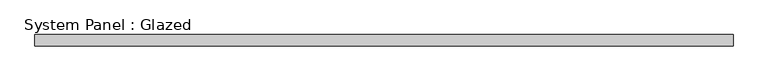
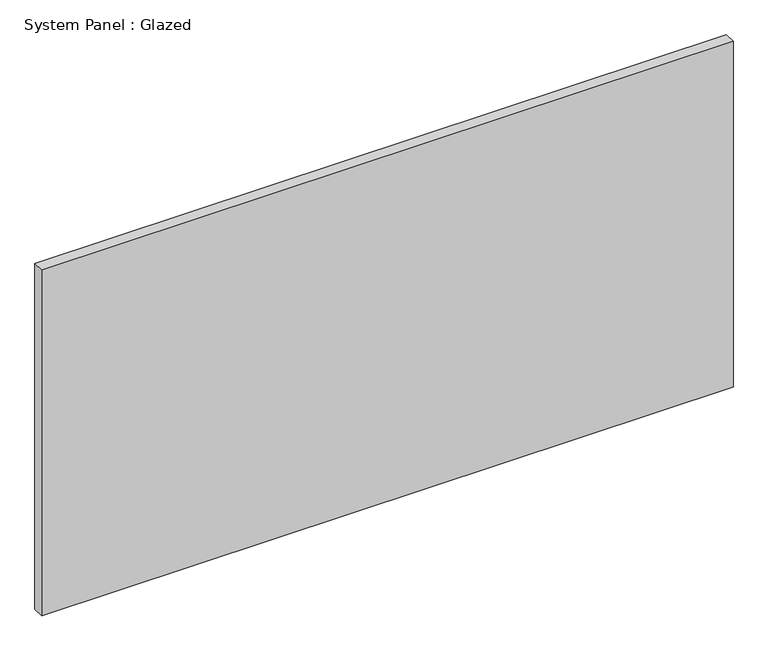
"""IFC4 building model written with IfcOpenShell, lengths in millimetres: plate geometry, System Panel : Glazed."""

import ifcopenshell
import ifcopenshell.guid

model = None  # the IFC model being written
_history = None  # IfcOwnerHistory: only IFC2X3 demands one
_inside = {}  # id of a spatial element -> (the spatial element, [elements in it])
_under = {}  # id of a project, library or spatial element -> (it, [spatial elements below it])
_declared = {}  # id of a project -> (the project, [libraries it declares])
_typed = {}  # id of a type object -> (the type object, [elements of that type])
_made_of = {}  # id of a material, layer set ... -> (it, [elements and type objects made of it])


def new_model(schema):
    """Start an empty IFC model of exactly this schema.

    Asked for "IFC4X3", IfcOpenShell would pick the latest addendum, in which some entities
    have other attributes; the version numbers below select the first issue.
    IFC2X3 requires an IfcOwnerHistory on every rooted entity: one is made here for all.
    """
    global model, _history
    if schema == "IFC4X3":
        model = ifcopenshell.file(schema_version=(4, 3, 0, 0))
    else:
        model = ifcopenshell.file(schema=schema)
    _inside.clear()
    _under.clear()
    _declared.clear()
    _typed.clear()
    _made_of.clear()
    _history = None
    if model.schema == "IFC2X3":
        org = make("IfcOrganization", Name="unknown")
        user = make(
            "IfcPersonAndOrganization",
            ThePerson=make("IfcPerson", FamilyName="unknown"),
            TheOrganization=org,
        )
        app = make(
            "IfcApplication",
            ApplicationDeveloper=org,
            Version="unknown",
            ApplicationFullName="unknown",
            ApplicationIdentifier="unknown",
        )
        _history = make(
            "IfcOwnerHistory",
            OwningUser=user,
            OwningApplication=app,
            ChangeAction="ADDED",
            CreationDate=0,
        )
    return model


def make(cls, **values):
    """One entity of the class cls with the attributes given. An attribute that is None is left unset."""
    return model.create_entity(
        cls, **{name: value for name, value in values.items() if value is not None}
    )


def rooted(cls, **values):
    """An entity with a GlobalId (a new one), such as an element, a storey or a relation."""
    return make(cls, GlobalId=ifcopenshell.guid.new(), OwnerHistory=_history, **values)


def si_unit(unit_type, name, prefix=None):
    """IfcSIUnit, for example si_unit("LENGTHUNIT", "METRE", prefix="MILLI")."""
    return make("IfcSIUnit", UnitType=unit_type, Prefix=prefix, Name=name)


def assignment(units):
    """IfcUnitAssignment: the units of a project."""
    return None if units is None else make("IfcUnitAssignment", Units=units)


def point(xyz):
    """IfcCartesianPoint."""
    return None if xyz is None else make("IfcCartesianPoint", Coordinates=xyz)


def direction(xyz):
    """IfcDirection."""
    return None if xyz is None else make("IfcDirection", DirectionRatios=xyz)


def frame(location, z_axis=None, x_axis=None):
    """IfcAxis2Placement3D, a coordinate frame: its origin and axes. An axis left out is left unset."""
    return make(
        "IfcAxis2Placement3D",
        Location=point(location),
        Axis=direction(z_axis),
        RefDirection=direction(x_axis),
    )


def origin():
    """The frame at (0, 0, 0) with its axes left unset."""
    return frame((0.0, 0.0, 0.0))


def origin_with_axes():
    """The frame at (0, 0, 0) with the z axis (0, 0, 1) and the x axis (1, 0, 0) written out."""
    return frame((0.0, 0.0, 0.0), z_axis=(0.0, 0.0, 1.0), x_axis=(1.0, 0.0, 0.0))


def place(relative_to, where):
    """IfcLocalPlacement: puts the frame where relative to a parent placement (None: the world)."""
    return make(
        "IfcLocalPlacement", PlacementRelTo=relative_to, RelativePlacement=where
    )


def context(
    kind, dimensions, precision=None, world=None, true_north=None, identifier=None
):
    """IfcGeometricRepresentationContext, for example the 3D "Model" context."""
    return make(
        "IfcGeometricRepresentationContext",
        ContextIdentifier=identifier,
        ContextType=kind,
        CoordinateSpaceDimension=dimensions,
        Precision=precision,
        WorldCoordinateSystem=world,
        TrueNorth=true_north,
    )


def project(units=None, contexts=None):
    """IfcProject with its units and contexts."""
    return rooted(
        "IfcProject",
        Name="project",
        RepresentationContexts=contexts,
        UnitsInContext=assignment(units),
    )


def spatial(cls, under=None, at=None, **own):
    """A site, building, storey or space (cls), placed at a placement, below another one or the project."""
    s = rooted(cls, ObjectPlacement=at, **own)
    if under is not None:
        _under.setdefault(under.id(), (under, []))[1].append(s)
    return s


def polyline(points):
    """IfcPolyline through the points."""
    return make("IfcPolyline", Points=[point(p) for p in points])


def outline(outer, holes=None, kind="AREA"):
    """IfcArbitraryClosedProfileDef: a profile drawn as a closed curve; with holes, ...WithVoids."""
    if holes is None:
        return make("IfcArbitraryClosedProfileDef", ProfileType=kind, OuterCurve=outer)
    return make(
        "IfcArbitraryProfileDefWithVoids",
        ProfileType=kind,
        OuterCurve=outer,
        InnerCurves=holes,
    )


def extrude(swept, where, along, depth):
    """IfcExtrudedAreaSolid: the profile swept, set in the frame where, extruded along a direction by depth."""
    return make(
        "IfcExtrudedAreaSolid",
        SweptArea=swept,
        Position=where,
        ExtrudedDirection=direction(along),
        Depth=depth,
    )


def shape(context_of_items, identifier, shape_type, items):
    """IfcShapeRepresentation: the items that make up one representation, for example the "Body"."""
    return make(
        "IfcShapeRepresentation",
        ContextOfItems=context_of_items,
        RepresentationIdentifier=identifier,
        RepresentationType=shape_type,
        Items=items,
    )


def source(mapping_origin, context_of_items, identifier, shape_type, items):
    """IfcRepresentationMap: a shape defined once, which mapped items show again and again."""
    return make(
        "IfcRepresentationMap",
        MappingOrigin=mapping_origin,
        MappedRepresentation=shape(context_of_items, identifier, shape_type, items),
    )


def transform(
    local_origin,
    x_axis=None,
    y_axis=None,
    z_axis=None,
    scale=None,
    scale2=None,
    scale3=None,
    uniform=True,
):
    """IfcCartesianTransformationOperator3D, or its non-uniform kind. x_axis, y_axis, z_axis: its Axis1, 2, 3."""
    if uniform:
        return make(
            "IfcCartesianTransformationOperator3D",
            Axis1=direction(x_axis),
            Axis2=direction(y_axis),
            LocalOrigin=point(local_origin),
            Scale=scale,
            Axis3=direction(z_axis),
        )
    return make(
        "IfcCartesianTransformationOperator3DnonUniform",
        Axis1=direction(x_axis),
        Axis2=direction(y_axis),
        LocalOrigin=point(local_origin),
        Scale=scale,
        Axis3=direction(z_axis),
        Scale2=scale2,
        Scale3=scale3,
    )


def mapped(mapping_source, mapping_target):
    """IfcMappedItem: shows the shape of a source again, moved by a transform."""
    return make(
        "IfcMappedItem", MappingSource=mapping_source, MappingTarget=mapping_target
    )


def made_of(thing, what):
    """Note that an element or type object is made of a material, layer set ...; save() writes the relation."""
    if what is not None:
        _made_of.setdefault(what.id(), (what, []))[1].append(thing)
    return thing


def element(
    cls,
    number,
    at=None,
    inside=None,
    cuts=None,
    type_object=None,
    material=None,
    context=None,
    identifier="Body",
    shape_type=None,
    held_by="IfcProductDefinitionShape",
    body=None,
    shapes=None,
    **own,
):
    """One element of the class cls, such as IfcWall. Its Tag is "e" and its number.

    at: its placement. inside: the storey or other place that contains it. cuts: it is an
    opening in that element (IfcRelVoidsElement). A single representation is given by context,
    identifier, shape_type and body (its items); several are given by shapes. held_by: the class
    of the entity that holds the representations. save() writes the other relations.
    """
    e = rooted(cls, Tag="e%d" % number, ObjectPlacement=at, **own)
    if body is not None:
        shapes = [shape(context, identifier, shape_type, body)]
    if shapes is not None:
        e.Representation = make(held_by, Representations=shapes)
    if inside is not None:
        _inside.setdefault(inside.id(), (inside, []))[1].append(e)
    if cuts is not None:
        rooted(
            "IfcRelVoidsElement", RelatingBuildingElement=cuts, RelatedOpeningElement=e
        )
    if type_object is not None:
        _typed.setdefault(type_object.id(), (type_object, []))[1].append(e)
    return made_of(e, material)


def aggregate(whole, parts):
    """IfcRelAggregates: a whole, such as a stair, and the parts it consists of."""
    return rooted("IfcRelAggregates", RelatingObject=whole, RelatedObjects=parts)


def save(model, path):
    """Write the relations noted so far, then the file.

    IfcRelAggregates (storeys below a building ...), IfcRelContainedInSpatialStructure (elements
    in a storey), IfcRelDefinesByType, IfcRelAssociatesMaterial and IfcRelDeclares: one each for
    every whole, place, type object, material and project.
    """
    for whole, parts in _under.values():
        aggregate(whole, parts)
    for where, things in _inside.values():
        rooted(
            "IfcRelContainedInSpatialStructure",
            RelatedElements=things,
            RelatingStructure=where,
        )
    for kind, things in _typed.values():
        rooted("IfcRelDefinesByType", RelatedObjects=things, RelatingType=kind)
    for what, things in _made_of.values():
        rooted("IfcRelAssociatesMaterial", RelatedObjects=things, RelatingMaterial=what)
    for by, libraries in _declared.values():
        rooted("IfcRelDeclares", RelatingContext=by, RelatedDefinitions=libraries)
    model.write(path)


def system_panel_glazed_a79b8077(model_context):
    return source(origin(), model_context, "Body", "SweptSolid", [
        extrude(outline(polyline([(768.3500002, -44.45), (-768.3500002, -44.45), (-768.3500002, -19.05), (768.3500002, -19.05), (768.3500002, -44.45)])), origin_with_axes(), (0.0, 0.0, 1.0), 812.8),
    ])


if __name__ == "__main__":
    model = new_model("IFC4")
    model_context = context("Model", 3, world=origin())
    ifc_project = project(units=[si_unit("LENGTHUNIT", "METRE", prefix="MILLI")], contexts=[model_context])
    site = spatial("IfcSite", under=ifc_project)
    building = spatial("IfcBuilding", under=site)
    placement = place(None, origin())
    system_panel_glazed_shape = system_panel_glazed_a79b8077(model_context)
    element("IfcPlate", 1, ObjectType="System Panel : Glazed", at=placement, inside=building, context=model_context, shape_type="MappedRepresentation", body=[
        mapped(system_panel_glazed_shape, transform((0.0, 0.0, 0.0), x_axis=(1.0, 0.0, 0.0), y_axis=(0.0, 1.0, 0.0), z_axis=(0.0, 0.0, 1.0))),
    ])
    save(model, "model.ifc")

# Revit data of these elements
# Element 1 (IfcPlate, "System Panel : Glazed")
#   Materials on its faces: "Glass"
# Materials
#   "Glass": class "Glass", colour RGB 0 128 192, transparency 0.75
